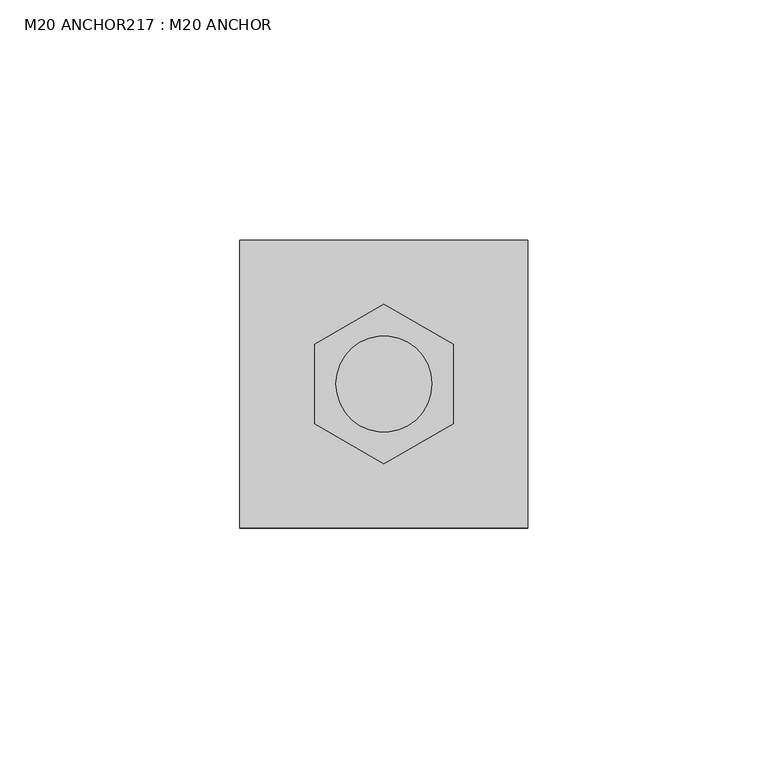
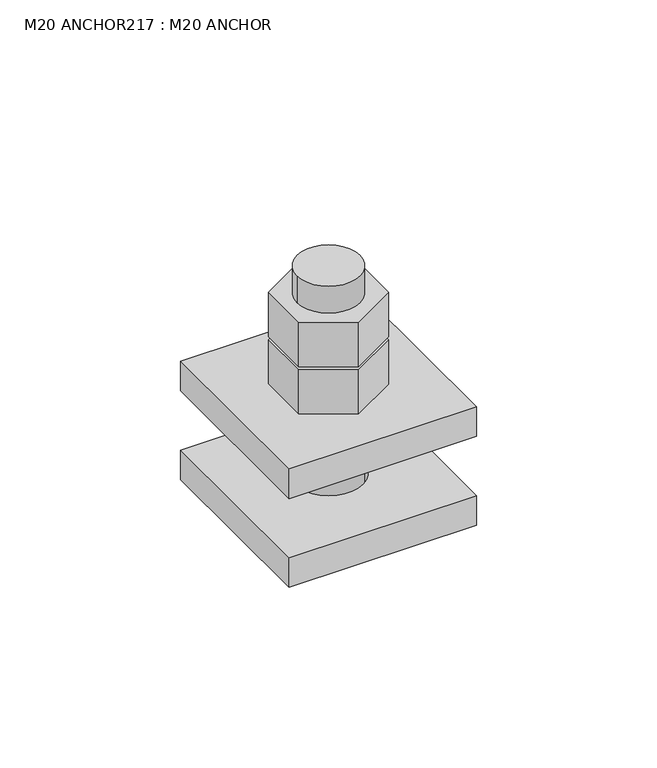
"""IFC4 building model written with IfcOpenShell, lengths in millimetres: fastener geometry, M20 ANCHOR217 : M20 ANCHOR."""

from ifc_helpers import new_model, si_unit, point, frame, frame_2d, origin, place, context, project, spatial, polyline, circle_curve, trimmed, segment, composite_curve, outline, extrude, source, transform, mapped, element, save


def m20_anchor217_m20_anchor_cce4f45e(model_context):
    return source(origin(), model_context, "Body", "SweptSolid", [
        extrude(outline(polyline([(8991.9144032, 25545.0952779), (8991.9144032, 25528.4582151), (8977.5062842, 25520.1396837), (8963.0981652, 25528.4582151), (8963.0981652, 25545.0952779), (8977.5062842, 25553.4138093), (8991.9144032, 25545.0952779)]), holes=[composite_curve([segment(trimmed(circle_curve(frame_2d((8977.5062842, 25536.7767465)), 10.0), [point((8967.5062842, 25536.7767465))], [point((8987.5062842, 25536.7767465))], True, "CARTESIAN"), True, "CONTINUOUS"), segment(trimmed(circle_curve(frame_2d((8977.5062842, 25536.7767465)), 10.0), [point((8987.5062842, 25536.7767465))], [point((8967.5062842, 25536.7767465))], True, "CARTESIAN"), True, "CONTINUOUS")], self_intersect=False)]), frame((0.0, 0.0, 246.0), z_axis=(0.0, 0.0, 1.0), x_axis=(1.0, 0.0, 0.0)), (0.0, 0.0, 1.0), 15.0),
        extrude(outline(polyline([(8991.9144032, 25545.0952779), (8991.9144032, 25528.4582151), (8977.5062842, 25520.1396837), (8963.0981652, 25528.4582151), (8963.0981652, 25545.0952779), (8977.5062842, 25553.4138093), (8991.9144032, 25545.0952779)]), holes=[composite_curve([segment(trimmed(circle_curve(frame_2d((8977.5062842, 25536.7767465)), 10.0), [point((8967.5062842, 25536.7767465))], [point((8987.5062842, 25536.7767465))], True, "CARTESIAN"), True, "CONTINUOUS"), segment(trimmed(circle_curve(frame_2d((8977.5062842, 25536.7767465)), 10.0), [point((8987.5062842, 25536.7767465))], [point((8967.5062842, 25536.7767465))], True, "CARTESIAN"), True, "CONTINUOUS")], self_intersect=False)]), frame((0.0, 0.0, 230.0), z_axis=(0.0, 0.0, 1.0), x_axis=(1.0, 0.0, 0.0)), (0.0, 0.0, 1.0), 15.0),
        extrude(outline(composite_curve([segment(trimmed(circle_curve(frame_2d((8977.5062842, 25536.7767465)), 10.0), [point((8967.5062842, 25536.7767465))], [point((8987.5062842, 25536.7767465))], False, "CARTESIAN"), True, "CONTINUOUS"), segment(trimmed(circle_curve(frame_2d((8977.5062842, 25536.7767465)), 10.0), [point((8987.5062842, 25536.7767465))], [point((8967.5062842, 25536.7767465))], False, "CARTESIAN"), True, "CONTINUOUS")], self_intersect=False)), frame((0.0, 0.0, 190.0), z_axis=(0.0, 0.0, 1.0), x_axis=(1.0, 0.0, 0.0)), (0.0, 0.0, 1.0), 80.0),
        extrude(outline(polyline([(9007.5062842, 25566.7767465), (9007.5062842, 25506.7767465), (8947.5062842, 25506.7767465), (8947.5062842, 25566.7767465), (9007.5062842, 25566.7767465)]), holes=[composite_curve([segment(trimmed(circle_curve(frame_2d((8977.5062842, 25536.7767465)), 11.0), [point((8966.5062842, 25536.7767465))], [point((8988.5062842, 25536.7767465))], True, "CARTESIAN"), True, "CONTINUOUS"), segment(trimmed(circle_curve(frame_2d((8977.5062842, 25536.7767465)), 11.0), [point((8988.5062842, 25536.7767465))], [point((8966.5062842, 25536.7767465))], True, "CARTESIAN"), True, "CONTINUOUS")], self_intersect=False)]), frame((0.0, 0.0, 190.0), z_axis=(0.0, 0.0, 1.0), x_axis=(1.0, 0.0, 0.0)), (0.0, 0.0, 1.0), 10.0),
        extrude(outline(polyline([(9007.5062842, 25566.7767465), (9007.5062842, 25506.7767465), (8947.5062842, 25506.7767465), (8947.5062842, 25566.7767465), (9007.5062842, 25566.7767465)]), holes=[composite_curve([segment(trimmed(circle_curve(frame_2d((8977.5062842, 25536.7767465)), 11.0), [point((8966.5062842, 25536.7767465))], [point((8988.5062842, 25536.7767465))], True, "CARTESIAN"), True, "CONTINUOUS"), segment(trimmed(circle_curve(frame_2d((8977.5062842, 25536.7767465)), 11.0), [point((8988.5062842, 25536.7767465))], [point((8966.5062842, 25536.7767465))], True, "CARTESIAN"), True, "CONTINUOUS")], self_intersect=False)]), frame((0.0, 0.0, 220.0), z_axis=(0.0, 0.0, 1.0), x_axis=(1.0, 0.0, 0.0)), (0.0, 0.0, 1.0), 10.0),
    ])


if __name__ == "__main__":
    model = new_model("IFC4")
    model_context = context("Model", 3, world=origin())
    ifc_project = project(units=[si_unit("LENGTHUNIT", "METRE", prefix="MILLI")], contexts=[model_context])
    site = spatial("IfcSite", under=ifc_project)
    building = spatial("IfcBuilding", under=site)
    placement = place(None, origin())
    m20_anchor217_m20_anchor_shape = m20_anchor217_m20_anchor_cce4f45e(model_context)
    element("IfcFastener", 1, ObjectType="M20 ANCHOR217 : M20 ANCHOR", at=placement, inside=building, context=model_context, shape_type="MappedRepresentation", body=[
        mapped(m20_anchor217_m20_anchor_shape, transform((0.0, 0.0, 0.0), x_axis=(1.0, 0.0, 0.0), y_axis=(0.0, 1.0, 0.0), z_axis=(0.0, 0.0, 1.0))),
    ])
    save(model, "model.ifc")
